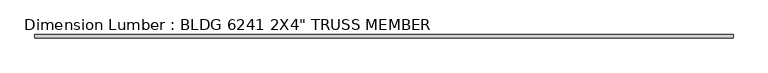
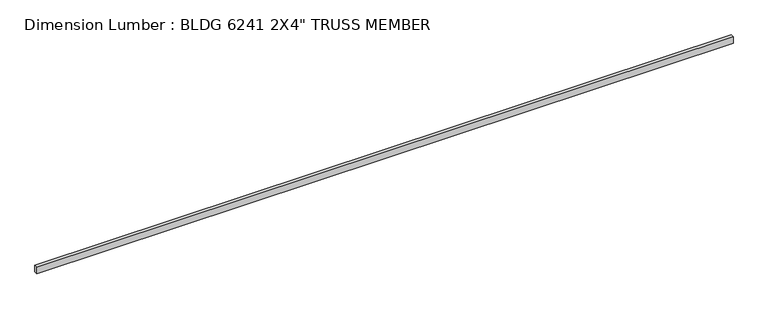
"""IFC4 building model written with IfcOpenShell, lengths in millimetres: beam geometry."""

from ifc_helpers import new_model, si_unit, frame, origin, place, context, project, spatial, polyline, outline, extrude, source, transform, mapped, element, save


def beam_a4242642(model_context):
    return source(origin(), model_context, "Body", "SweptSolid", [
        extrude(outline(polyline([(5145.3336481, 25.4), (5145.3336481, -25.4), (-5145.3336481, -25.4), (-5145.3336481, 25.4), (5145.3336481, 25.4)])), frame((0.0, 0.0, -50.8), z_axis=(0.0, 0.0, 1.0), x_axis=(1.0, 0.0, 0.0)), (0.0, 0.0, 1.0), 101.6),
    ])


if __name__ == "__main__":
    model = new_model("IFC4")
    model_context = context("Model", 3, world=origin())
    ifc_project = project(units=[si_unit("LENGTHUNIT", "METRE", prefix="MILLI")], contexts=[model_context])
    site = spatial("IfcSite", under=ifc_project)
    building = spatial("IfcBuilding", under=site)
    placement = place(None, origin())
    beam_shape = beam_a4242642(model_context)
    element("IfcBeam", 1, ObjectType="Dimension Lumber : BLDG 6241 2X4\" TRUSS MEMBER", at=placement, inside=building, context=model_context, shape_type="MappedRepresentation", body=[
        mapped(beam_shape, transform((0.0, 0.0, 0.0), x_axis=(1.0, 0.0, 0.0), y_axis=(0.0, 1.0, 0.0), z_axis=(0.0, 0.0, 1.0))),
    ])
    save(model, "model.ifc")

# Revit data of these elements
# Type "Dimension Lumber : BLDG 6241 2X4\" TRUSS MEMBER"
#   Assembly Code = "B10"
#   A = 0.273472 SF
#   Length [instance default] = 5' - 0"
#   b = 0' - 2"
#   d = 0' - 4"
#   Structural Material [instance default] = Softwood, Lumber
# Element 1 (IfcBeam, "Dimension Lumber : BLDG 6241 2X4\" TRUSS MEMBER")
#   Materials on its faces: "Softwood, Lumber"
# Materials
#   "Softwood, Lumber": class "Wood", colour RGB 223 192 134, transparency 0, Description = "Pinus Echinata", Cost = 0
